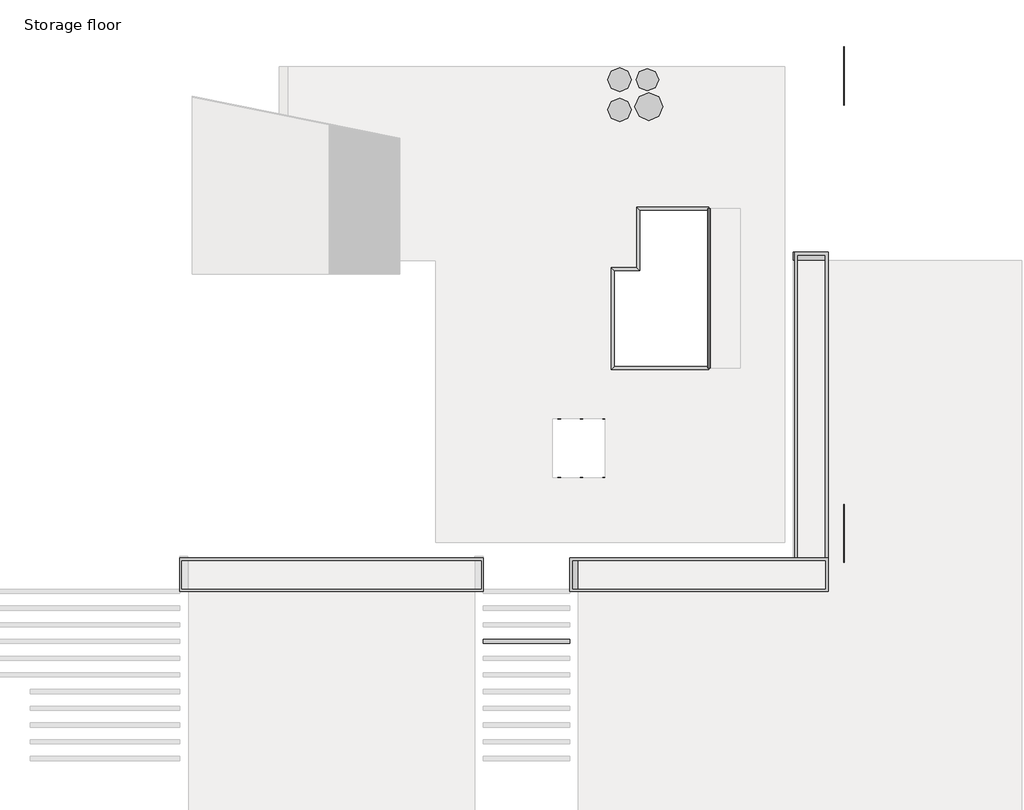
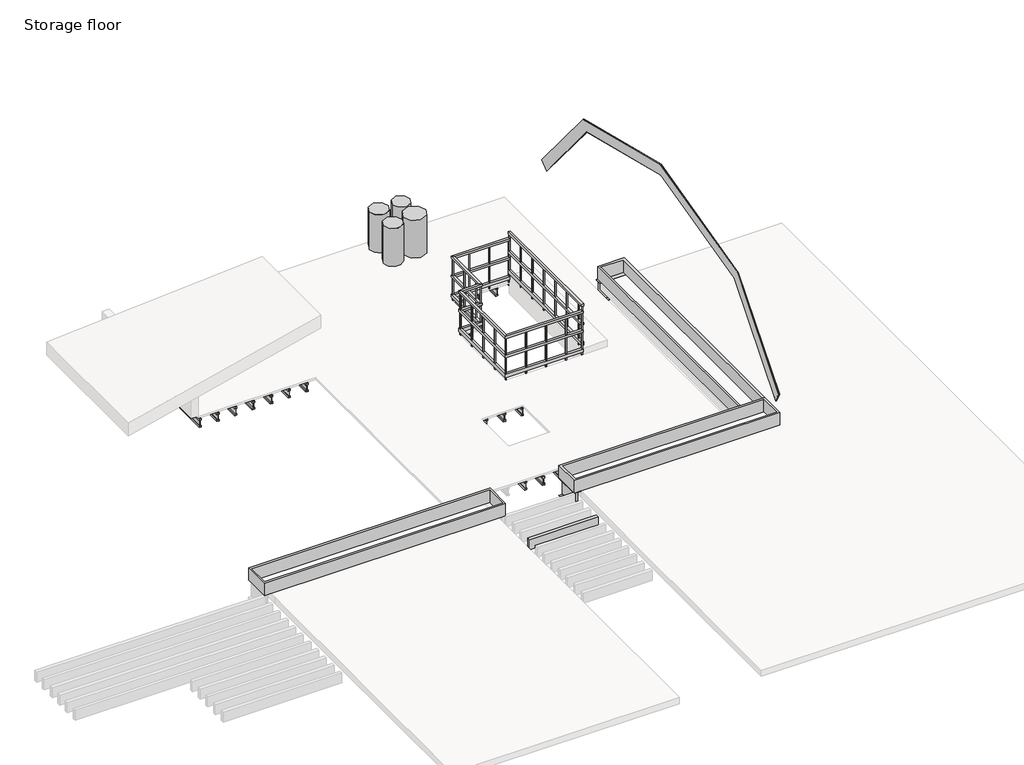
# One storey, part 2 of 2: 29 beams, 9 proxies, 2 railings.
"""IFC4 building model written with IfcOpenShell, lengths in millimetres."""

import ifcopenshell
import ifcopenshell.guid

model = None  # the IFC model being written
_history = None  # IfcOwnerHistory: only IFC2X3 demands one
_inside = {}  # id of a spatial element -> (the spatial element, [elements in it])
_under = {}  # id of a project, library or spatial element -> (it, [spatial elements below it])
_declared = {}  # id of a project -> (the project, [libraries it declares])
_typed = {}  # id of a type object -> (the type object, [elements of that type])
_made_of = {}  # id of a material, layer set ... -> (it, [elements and type objects made of it])


def new_model(schema):
    """Start an empty IFC model of exactly this schema.

    Asked for "IFC4X3", IfcOpenShell would pick the latest addendum, in which some entities
    have other attributes; the version numbers below select the first issue.
    IFC2X3 requires an IfcOwnerHistory on every rooted entity: one is made here for all.
    """
    global model, _history
    if schema == "IFC4X3":
        model = ifcopenshell.file(schema_version=(4, 3, 0, 0))
    else:
        model = ifcopenshell.file(schema=schema)
    _inside.clear()
    _under.clear()
    _declared.clear()
    _typed.clear()
    _made_of.clear()
    _history = None
    if model.schema == "IFC2X3":
        org = make("IfcOrganization", Name="unknown")
        user = make(
            "IfcPersonAndOrganization",
            ThePerson=make("IfcPerson", FamilyName="unknown"),
            TheOrganization=org,
        )
        app = make(
            "IfcApplication",
            ApplicationDeveloper=org,
            Version="unknown",
            ApplicationFullName="unknown",
            ApplicationIdentifier="unknown",
        )
        _history = make(
            "IfcOwnerHistory",
            OwningUser=user,
            OwningApplication=app,
            ChangeAction="ADDED",
            CreationDate=0,
        )
    return model


def make(cls, **values):
    """One entity of the class cls with the attributes given. An attribute that is None is left unset."""
    return model.create_entity(
        cls, **{name: value for name, value in values.items() if value is not None}
    )


def rooted(cls, **values):
    """An entity with a GlobalId (a new one), such as an element, a storey or a relation."""
    return make(cls, GlobalId=ifcopenshell.guid.new(), OwnerHistory=_history, **values)


def si_unit(unit_type, name, prefix=None):
    """IfcSIUnit, for example si_unit("LENGTHUNIT", "METRE", prefix="MILLI")."""
    return make("IfcSIUnit", UnitType=unit_type, Prefix=prefix, Name=name)


def assignment(units):
    """IfcUnitAssignment: the units of a project."""
    return None if units is None else make("IfcUnitAssignment", Units=units)


def point(xyz):
    """IfcCartesianPoint."""
    return None if xyz is None else make("IfcCartesianPoint", Coordinates=xyz)


def direction(xyz):
    """IfcDirection."""
    return None if xyz is None else make("IfcDirection", DirectionRatios=xyz)


def frame(location, z_axis=None, x_axis=None):
    """IfcAxis2Placement3D, a coordinate frame: its origin and axes. An axis left out is left unset."""
    return make(
        "IfcAxis2Placement3D",
        Location=point(location),
        Axis=direction(z_axis),
        RefDirection=direction(x_axis),
    )


def frame_2d(location, x_axis=None):
    """IfcAxis2Placement2D, a coordinate frame in the plane: its origin and x axis."""
    return make(
        "IfcAxis2Placement2D", Location=point(location), RefDirection=direction(x_axis)
    )


def origin():
    """The frame at (0, 0, 0) with its axes left unset."""
    return frame((0.0, 0.0, 0.0))


def place(relative_to, where):
    """IfcLocalPlacement: puts the frame where relative to a parent placement (None: the world)."""
    return make(
        "IfcLocalPlacement", PlacementRelTo=relative_to, RelativePlacement=where
    )


def context(
    kind, dimensions, precision=None, world=None, true_north=None, identifier=None
):
    """IfcGeometricRepresentationContext, for example the 3D "Model" context."""
    return make(
        "IfcGeometricRepresentationContext",
        ContextIdentifier=identifier,
        ContextType=kind,
        CoordinateSpaceDimension=dimensions,
        Precision=precision,
        WorldCoordinateSystem=world,
        TrueNorth=true_north,
    )


def project(units=None, contexts=None):
    """IfcProject with its units and contexts."""
    return rooted(
        "IfcProject",
        Name="project",
        RepresentationContexts=contexts,
        UnitsInContext=assignment(units),
    )


def spatial(cls, under=None, at=None, **own):
    """A site, building, storey or space (cls), placed at a placement, below another one or the project."""
    s = rooted(cls, ObjectPlacement=at, **own)
    if under is not None:
        _under.setdefault(under.id(), (under, []))[1].append(s)
    return s


def polyline(points):
    """IfcPolyline through the points."""
    return make("IfcPolyline", Points=[point(p) for p in points])


def circle_curve(where, radius):
    """IfcCircle in the frame where."""
    return make("IfcCircle", Position=where, Radius=radius)


def trimmed(basis, trim1, trim2, sense, master):
    """IfcTrimmedCurve: the piece of a basis curve between two trims."""
    return make(
        "IfcTrimmedCurve",
        BasisCurve=basis,
        Trim1=trim1,
        Trim2=trim2,
        SenseAgreement=sense,
        MasterRepresentation=master,
    )


def segment(curve, same_sense, transition):
    """IfcCompositeCurveSegment."""
    return make(
        "IfcCompositeCurveSegment",
        Transition=transition,
        SameSense=same_sense,
        ParentCurve=curve,
    )


def composite_curve(segments, self_intersect=None):
    """IfcCompositeCurve: segments joined end to end."""
    return make("IfcCompositeCurve", Segments=segments, SelfIntersect=self_intersect)


def outline(outer, holes=None, kind="AREA"):
    """IfcArbitraryClosedProfileDef: a profile drawn as a closed curve; with holes, ...WithVoids."""
    if holes is None:
        return make("IfcArbitraryClosedProfileDef", ProfileType=kind, OuterCurve=outer)
    return make(
        "IfcArbitraryProfileDefWithVoids",
        ProfileType=kind,
        OuterCurve=outer,
        InnerCurves=holes,
    )


def extrude(swept, where, along, depth):
    """IfcExtrudedAreaSolid: the profile swept, set in the frame where, extruded along a direction by depth."""
    return make(
        "IfcExtrudedAreaSolid",
        SweptArea=swept,
        Position=where,
        ExtrudedDirection=direction(along),
        Depth=depth,
    )


def faces_of(points, faces, orient=None, outer=None):
    """IfcFace entities. A face is a list of loops; a loop is a list of indices into points, from 0.

    orient and outer hold one flag for each loop. By default every Orientation is true, the
    first loop of a face is its IfcFaceOuterBound and the others are IfcFaceBound.
    """
    made = []
    for i, loops in enumerate(faces):
        bounds = []
        for j, loop in enumerate(loops):
            is_outer = j == 0 if outer is None else outer[i][j]
            bounds.append(
                make(
                    "IfcFaceOuterBound" if is_outer else "IfcFaceBound",
                    Bound=make("IfcPolyLoop", Polygon=[points[k] for k in loop]),
                    Orientation=True if orient is None else orient[i][j],
                )
            )
        made.append(make("IfcFace", Bounds=bounds))
    return made


def faceted_brep(points, faces, orient=None, outer=None, voids=None):
    """IfcFacetedBrep: a solid bounded by flat faces; with voids (closed shells), ...WithVoids."""
    shared = [point(p) for p in points]
    hull = make("IfcClosedShell", CfsFaces=faces_of(shared, faces, orient, outer))
    if voids is None:
        return make("IfcFacetedBrep", Outer=hull)
    return make(
        "IfcFacetedBrepWithVoids",
        Outer=hull,
        Voids=[
            make(cls, CfsFaces=faces_of(shared, fs, o, b)) for cls, fs, o, b in voids
        ],
    )


def shape(context_of_items, identifier, shape_type, items):
    """IfcShapeRepresentation: the items that make up one representation, for example the "Body"."""
    return make(
        "IfcShapeRepresentation",
        ContextOfItems=context_of_items,
        RepresentationIdentifier=identifier,
        RepresentationType=shape_type,
        Items=items,
    )


def source(mapping_origin, context_of_items, identifier, shape_type, items):
    """IfcRepresentationMap: a shape defined once, which mapped items show again and again."""
    return make(
        "IfcRepresentationMap",
        MappingOrigin=mapping_origin,
        MappedRepresentation=shape(context_of_items, identifier, shape_type, items),
    )


def transform(
    local_origin,
    x_axis=None,
    y_axis=None,
    z_axis=None,
    scale=None,
    scale2=None,
    scale3=None,
    uniform=True,
):
    """IfcCartesianTransformationOperator3D, or its non-uniform kind. x_axis, y_axis, z_axis: its Axis1, 2, 3."""
    if uniform:
        return make(
            "IfcCartesianTransformationOperator3D",
            Axis1=direction(x_axis),
            Axis2=direction(y_axis),
            LocalOrigin=point(local_origin),
            Scale=scale,
            Axis3=direction(z_axis),
        )
    return make(
        "IfcCartesianTransformationOperator3DnonUniform",
        Axis1=direction(x_axis),
        Axis2=direction(y_axis),
        LocalOrigin=point(local_origin),
        Scale=scale,
        Axis3=direction(z_axis),
        Scale2=scale2,
        Scale3=scale3,
    )


def mapped(mapping_source, mapping_target):
    """IfcMappedItem: shows the shape of a source again, moved by a transform."""
    return make(
        "IfcMappedItem", MappingSource=mapping_source, MappingTarget=mapping_target
    )


def made_of(thing, what):
    """Note that an element or type object is made of a material, layer set ...; save() writes the relation."""
    if what is not None:
        _made_of.setdefault(what.id(), (what, []))[1].append(thing)
    return thing


def element(
    cls,
    number,
    at=None,
    inside=None,
    cuts=None,
    type_object=None,
    material=None,
    context=None,
    identifier="Body",
    shape_type=None,
    held_by="IfcProductDefinitionShape",
    body=None,
    shapes=None,
    **own,
):
    """One element of the class cls, such as IfcWall. Its Tag is "e" and its number.

    at: its placement. inside: the storey or other place that contains it. cuts: it is an
    opening in that element (IfcRelVoidsElement). A single representation is given by context,
    identifier, shape_type and body (its items); several are given by shapes. held_by: the class
    of the entity that holds the representations. save() writes the other relations.
    """
    e = rooted(cls, Tag="e%d" % number, ObjectPlacement=at, **own)
    if body is not None:
        shapes = [shape(context, identifier, shape_type, body)]
    if shapes is not None:
        e.Representation = make(held_by, Representations=shapes)
    if inside is not None:
        _inside.setdefault(inside.id(), (inside, []))[1].append(e)
    if cuts is not None:
        rooted(
            "IfcRelVoidsElement", RelatingBuildingElement=cuts, RelatedOpeningElement=e
        )
    if type_object is not None:
        _typed.setdefault(type_object.id(), (type_object, []))[1].append(e)
    return made_of(e, material)


def aggregate(whole, parts):
    """IfcRelAggregates: a whole, such as a stair, and the parts it consists of."""
    return rooted("IfcRelAggregates", RelatingObject=whole, RelatedObjects=parts)


def save(model, path):
    """Write the relations noted so far, then the file.

    IfcRelAggregates (storeys below a building ...), IfcRelContainedInSpatialStructure (elements
    in a storey), IfcRelDefinesByType, IfcRelAssociatesMaterial and IfcRelDeclares: one each for
    every whole, place, type object, material and project.
    """
    for whole, parts in _under.values():
        aggregate(whole, parts)
    for where, things in _inside.values():
        rooted(
            "IfcRelContainedInSpatialStructure",
            RelatedElements=things,
            RelatingStructure=where,
        )
    for kind, things in _typed.values():
        rooted("IfcRelDefinesByType", RelatedObjects=things, RelatingType=kind)
    for what, things in _made_of.values():
        rooted("IfcRelAssociatesMaterial", RelatedObjects=things, RelatingMaterial=what)
    for by, libraries in _declared.values():
        rooted("IfcRelDeclares", RelatingContext=by, RelatedDefinitions=libraries)
    model.write(path)


def plywood_web_joist_2_x_8_7c958bd9(model_context):
    return source(origin(), model_context, "Body", "SweptSolid", [
        extrude(outline(polyline([(-25.4, 101.6), (25.4, 101.6), (25.4, 63.5), (4.7625, 63.5), (4.7625, 69.85), (-4.7625, 69.85), (-4.7625, 63.5), (-25.4, 63.5), (-25.4, 101.6)])), frame((-4318.0, 0.0, 0.0), z_axis=(1.0, 0.0, 0.0), x_axis=(0.0, 1.0, 0.0)), (0.0, 0.0, 1.0), 8636.0),
        extrude(outline(polyline([(25.4, -63.5), (25.4, -101.6), (-25.4, -101.6), (-25.4, -63.5), (-4.7625, -63.5), (-4.7625, -69.1160374), (4.7625, -69.1160374), (4.7625, -63.5), (25.4, -63.5)])), frame((-4318.0, 0.0, 0.0), z_axis=(1.0, 0.0, 0.0), x_axis=(0.0, 1.0, 0.0)), (0.0, 0.0, 1.0), 8636.0),
        extrude(outline(polyline([(4318.0, 4.7625), (4318.0, -4.7625), (-4318.0, -4.7625), (-4318.0, 4.7625), (4318.0, 4.7625)])), frame((0.0, 0.0, -69.1160374), z_axis=(0.0, 0.0, 1.0), x_axis=(1.0, 0.0, 0.0)), (0.0, 0.0, 1.0), 138.9660374),
    ])


def plywood_web_joist_2_x_8_e6685f11(model_context):
    return source(origin(), model_context, "Body", "SweptSolid", [
        extrude(outline(polyline([(-25.4, 101.6), (25.4, 101.6), (25.4, 63.5), (4.7625, 63.5), (4.7625, 69.85), (-4.7625, 69.85), (-4.7625, 63.5), (-25.4, 63.5), (-25.4, 101.6)])), frame((-1284.2875, 0.0, 0.0), z_axis=(1.0, 0.0, 0.0), x_axis=(0.0, 1.0, 0.0)), (0.0, 0.0, 1.0), 2568.575),
        extrude(outline(polyline([(25.4, -63.5), (25.4, -101.6), (-25.4, -101.6), (-25.4, -63.5), (-4.7625, -63.5), (-4.7625, -69.1160374), (4.7625, -69.1160374), (4.7625, -63.5), (25.4, -63.5)])), frame((-1284.2875, 0.0, 0.0), z_axis=(1.0, 0.0, 0.0), x_axis=(0.0, 1.0, 0.0)), (0.0, 0.0, 1.0), 2568.575),
        extrude(outline(polyline([(1284.2875, 4.7625), (1284.2875, -4.7625), (-1284.2875, -4.7625), (-1284.2875, 4.7625), (1284.2875, 4.7625)])), frame((0.0, 0.0, -69.1160374), z_axis=(0.0, 0.0, 1.0), x_axis=(1.0, 0.0, 0.0)), (0.0, 0.0, 1.0), 138.9660374),
    ])


def plywood_web_joist_2_x_8_5f52603e(model_context):
    return source(origin(), model_context, "Body", "SweptSolid", [
        extrude(outline(polyline([(-25.4, 101.6), (25.4, 101.6), (25.4, 63.5), (4.7625, 63.5), (4.7625, 69.85), (-4.7625, 69.85), (-4.7625, 63.5), (-25.4, 63.5), (-25.4, 101.6)])), frame((-1584.325, 0.0, 0.0), z_axis=(1.0, 0.0, 0.0), x_axis=(0.0, 1.0, 0.0)), (0.0, 0.0, 1.0), 3168.65),
        extrude(outline(polyline([(25.4, -63.5), (25.4, -101.6), (-25.4, -101.6), (-25.4, -63.5), (-4.7625, -63.5), (-4.7625, -69.1160374), (4.7625, -69.1160374), (4.7625, -63.5), (25.4, -63.5)])), frame((-1584.325, 0.0, 0.0), z_axis=(1.0, 0.0, 0.0), x_axis=(0.0, 1.0, 0.0)), (0.0, 0.0, 1.0), 3168.65),
        extrude(outline(polyline([(1584.325, 4.7625), (1584.325, -4.7625), (-1584.325, -4.7625), (-1584.325, 4.7625), (1584.325, 4.7625)])), frame((0.0, 0.0, -69.1160374), z_axis=(0.0, 0.0, 1.0), x_axis=(1.0, 0.0, 0.0)), (0.0, 0.0, 1.0), 138.9660374),
    ])


def plywood_web_joist_2_x_8_093a3c26(model_context):
    return source(origin(), model_context, "Body", "SweptSolid", [
        extrude(outline(polyline([(-25.4, 101.6), (25.4, 101.6), (25.4, 63.5), (4.7625, 63.5), (4.7625, 69.85), (-4.7625, 69.85), (-4.7625, 63.5), (-25.4, 63.5), (-25.4, 101.6)])), frame((-1835.15, 0.0, 0.0), z_axis=(1.0, 0.0, 0.0), x_axis=(0.0, 1.0, 0.0)), (0.0, 0.0, 1.0), 3670.3),
        extrude(outline(polyline([(25.4, -63.5), (25.4, -101.6), (-25.4, -101.6), (-25.4, -63.5), (-4.7625, -63.5), (-4.7625, -69.1160374), (4.7625, -69.1160374), (4.7625, -63.5), (25.4, -63.5)])), frame((-1835.15, 0.0, 0.0), z_axis=(1.0, 0.0, 0.0), x_axis=(0.0, 1.0, 0.0)), (0.0, 0.0, 1.0), 3670.3),
        extrude(outline(polyline([(1835.15, 4.7625), (1835.15, -4.7625), (-1835.15, -4.7625), (-1835.15, 4.7625), (1835.15, 4.7625)])), frame((0.0, 0.0, -69.1160374), z_axis=(0.0, 0.0, 1.0), x_axis=(1.0, 0.0, 0.0)), (0.0, 0.0, 1.0), 138.9660374),
    ])


def plywood_web_joist_2_x_8_156d774c(model_context):
    return source(origin(), model_context, "Body", "SweptSolid", [
        extrude(outline(polyline([(-25.4, 101.6), (25.4, 101.6), (25.4, 63.5), (4.7625, 63.5), (4.7625, 69.85), (-4.7625, 69.85), (-4.7625, 63.5), (-25.4, 63.5), (-25.4, 101.6)])), frame((-3195.5616975, 0.0, 0.0), z_axis=(1.0, 0.0, 0.0), x_axis=(0.0, 1.0, 0.0)), (0.0, 0.0, 1.0), 6391.1233951),
        extrude(outline(polyline([(25.4, -63.5), (25.4, -101.6), (-25.4, -101.6), (-25.4, -63.5), (-4.7625, -63.5), (-4.7625, -69.1160374), (4.7625, -69.1160374), (4.7625, -63.5), (25.4, -63.5)])), frame((-3195.5616975, 0.0, 0.0), z_axis=(1.0, 0.0, 0.0), x_axis=(0.0, 1.0, 0.0)), (0.0, 0.0, 1.0), 6391.1233951),
        extrude(outline(polyline([(3195.5616975, 4.7625), (3195.5616975, -4.7625), (-3195.5616975, -4.7625), (-3195.5616975, 4.7625), (3195.5616975, 4.7625)])), frame((0.0, 0.0, -69.1160374), z_axis=(0.0, 0.0, 1.0), x_axis=(1.0, 0.0, 0.0)), (0.0, 0.0, 1.0), 138.9660374),
    ])


def plywood_web_joist_2_x_8_69fe57bf(model_context):
    return source(origin(), model_context, "Body", "SweptSolid", [
        extrude(outline(polyline([(-25.4, 101.6), (25.4, 101.6), (25.4, 63.5), (4.7625, 63.5), (4.7625, 69.85), (-4.7625, 69.85), (-4.7625, 63.5), (-25.4, 63.5), (-25.4, 101.6)])), frame((-589.0383025, 0.0, 0.0), z_axis=(1.0, 0.0, 0.0), x_axis=(0.0, 1.0, 0.0)), (0.0, 0.0, 1.0), 1178.0766049),
        extrude(outline(polyline([(25.4, -63.5), (25.4, -101.6), (-25.4, -101.6), (-25.4, -63.5), (-4.7625, -63.5), (-4.7625, -69.1160374), (4.7625, -69.1160374), (4.7625, -63.5), (25.4, -63.5)])), frame((-589.0383025, 0.0, 0.0), z_axis=(1.0, 0.0, 0.0), x_axis=(0.0, 1.0, 0.0)), (0.0, 0.0, 1.0), 1178.0766049),
        extrude(outline(polyline([(589.0383025, 4.7625), (589.0383025, -4.7625), (-589.0383025, -4.7625), (-589.0383025, 4.7625), (589.0383025, 4.7625)])), frame((0.0, 0.0, -69.1160374), z_axis=(0.0, 0.0, 1.0), x_axis=(1.0, 0.0, 0.0)), (0.0, 0.0, 1.0), 138.9660374),
    ])


def plywood_web_joist_2_x_8_8e4157b3(model_context):
    return source(origin(), model_context, "Body", "SweptSolid", [
        extrude(outline(polyline([(-25.4, 101.6), (25.4, 101.6), (25.4, 63.5), (4.7625, 63.5), (4.7625, 69.85), (-4.7625, 69.85), (-4.7625, 63.5), (-25.4, 63.5), (-25.4, 101.6)])), frame((-1758.95, 0.0, 0.0), z_axis=(1.0, 0.0, 0.0), x_axis=(0.0, 1.0, 0.0)), (0.0, 0.0, 1.0), 3517.9),
        extrude(outline(polyline([(25.4, -63.5), (25.4, -101.6), (-25.4, -101.6), (-25.4, -63.5), (-4.7625, -63.5), (-4.7625, -69.1160374), (4.7625, -69.1160374), (4.7625, -63.5), (25.4, -63.5)])), frame((-1758.95, 0.0, 0.0), z_axis=(1.0, 0.0, 0.0), x_axis=(0.0, 1.0, 0.0)), (0.0, 0.0, 1.0), 3517.9),
        extrude(outline(polyline([(1758.95, 4.7625), (1758.95, -4.7625), (-1758.95, -4.7625), (-1758.95, 4.7625), (1758.95, 4.7625)])), frame((0.0, 0.0, -69.1160374), z_axis=(0.0, 0.0, 1.0), x_axis=(1.0, 0.0, 0.0)), (0.0, 0.0, 1.0), 138.9660374),
    ])


def timber_3x10_88a0bdfd(model_context):
    return source(origin(), model_context, "Body", "SweptSolid", [
        extrude(outline(polyline([(785.1325751, 38.1), (785.1325751, -38.1), (-785.1325751, -38.1), (-785.1325751, 38.1), (785.1325751, 38.1)])), frame((0.0, 0.0, -120.65), z_axis=(0.0, 0.0, 1.0), x_axis=(1.0, 0.0, 0.0)), (0.0, 0.0, 1.0), 241.3),
    ])


def w_shapes_w_6x16_3_4_ba0ed1b2(model_context):
    return source(origin(), model_context, "Body", "SweptSolid", [
        extrude(outline(composite_curve([segment(polyline([(76.1964281, -203.073), (76.1964281, -212.725), (-76.2035719, -212.725), (-76.2035719, -203.073), (-10.5445719, -203.073)]), True, "CONTINUOUS"), segment(trimmed(circle_curve(frame_2d((-10.5445719, -195.453)), 7.62), [point((-10.5445719, -203.073))], [point((-2.9245719, -195.453))], True, "CARTESIAN"), True, "CONTINUOUS"), segment(polyline([(-2.9245719, -195.453), (-2.9245719, 195.453)]), True, "CONTINUOUS"), segment(trimmed(circle_curve(frame_2d((-10.5445719, 195.453)), 7.62), [point((-2.9245719, 195.453))], [point((-10.5445719, 203.073))], True, "CARTESIAN"), True, "CONTINUOUS"), segment(polyline([(-10.5445719, 203.073), (-76.2035719, 203.073), (-76.2035719, 212.725), (76.1964281, 212.725), (76.1964281, 203.073), (10.5374281, 203.073)]), True, "CONTINUOUS"), segment(trimmed(circle_curve(frame_2d((10.5374281, 195.453)), 7.62), [point((10.5374281, 203.073))], [point((2.9174281, 195.453))], True, "CARTESIAN"), True, "CONTINUOUS"), segment(polyline([(2.9174281, 195.453), (2.9174281, -195.453)]), True, "CONTINUOUS"), segment(trimmed(circle_curve(frame_2d((10.5374281, -195.453)), 7.62), [point((2.9174281, -195.453))], [point((10.5374281, -203.073))], True, "CARTESIAN"), True, "CONTINUOUS"), segment(polyline([(10.5374281, -203.073), (76.1964281, -203.073)]), True, "CONTINUOUS")], self_intersect=False)), frame((-303.1556375, 0.0, 0.0), z_axis=(1.0, 0.0, 0.0), x_axis=(0.0, 1.0, 0.0)), (0.0, 0.0, 1.0), 606.311275),
    ])


def w_shapes_w_6x18_5_26640f6b(model_context):
    return source(origin(), model_context, "Body", "SweptSolid", [
        extrude(outline(composite_curve([segment(polyline([(76.1964281, -225.298), (76.1964281, -234.95), (-76.2035719, -234.95), (-76.2035719, -225.298), (-10.5445719, -225.298)]), True, "CONTINUOUS"), segment(trimmed(circle_curve(frame_2d((-10.5445719, -217.678)), 7.62), [point((-10.5445719, -225.298))], [point((-2.9245719, -217.678))], True, "CARTESIAN"), True, "CONTINUOUS"), segment(polyline([(-2.9245719, -217.678), (-2.9245719, 217.678)]), True, "CONTINUOUS"), segment(trimmed(circle_curve(frame_2d((-10.5445719, 217.678)), 7.62), [point((-2.9245719, 217.678))], [point((-10.5445719, 225.298))], True, "CARTESIAN"), True, "CONTINUOUS"), segment(polyline([(-10.5445719, 225.298), (-76.2035719, 225.298), (-76.2035719, 234.95), (76.1964281, 234.95), (76.1964281, 225.298), (10.5374281, 225.298)]), True, "CONTINUOUS"), segment(trimmed(circle_curve(frame_2d((10.5374281, 217.678)), 7.62), [point((10.5374281, 225.298))], [point((2.9174281, 217.678))], True, "CARTESIAN"), True, "CONTINUOUS"), segment(polyline([(2.9174281, 217.678), (2.9174281, -217.678)]), True, "CONTINUOUS"), segment(trimmed(circle_curve(frame_2d((10.5374281, -217.678)), 7.62), [point((2.9174281, -217.678))], [point((10.5374281, -225.298))], True, "CARTESIAN"), True, "CONTINUOUS"), segment(polyline([(10.5374281, -225.298), (76.1964281, -225.298)]), True, "CONTINUOUS")], self_intersect=False)), frame((-317.5, 0.0, 0.0), z_axis=(1.0, 0.0, 0.0), x_axis=(0.0, 1.0, 0.0)), (0.0, 0.0, 1.0), 635.0),
    ])


def generic_models_2_generic_models_1_059ed1a1(model_context):
    return source(origin(), model_context, "Body", "SweptSolid", [
        extrude(outline(polyline([(11609.9309883, 2984.3405795), (10023.6412719, 4887.8882391), (7113.0570149, 5615.5343034), (4202.4384941, 4887.8796732), (2560.7151338, 2917.8116409), (2434.8673967, 3148.0206952), (4066.3626163, 5105.8149588), (7113.772024, 5867.6673107), (10161.1814316, 5105.8149588), (11797.360301, 3142.4003155), (11609.9309883, 2984.3405795)])), frame((29947.3870052, 0.0, 0.0), z_axis=(1.0, 0.0, 0.0), x_axis=(0.0, 1.0, 0.0)), (0.0, 0.0, 1.0), 13.5023771),
    ])


def generic_models_4_generic_models_1_4f2df183(model_context):
    return source(origin(), model_context, "Body", "SweptSolid", [
        extrude(outline(polyline([(11606.2878096, 2984.3405795), (10019.9980933, 4887.8882391), (7109.4138362, 5615.5343034), (4198.7953154, 4887.8796732), (2604.5089175, 2974.7359957), (2431.2242181, 3148.0206952), (4062.7194377, 5105.8149588), (7110.1288453, 5867.6673107), (10157.5382529, 5105.8149588), (11793.7171223, 3142.4003155), (11606.2878096, 2984.3405795)])), frame((29947.3870052, 0.0, 0.0), z_axis=(1.0, 0.0, 0.0), x_axis=(0.0, 1.0, 0.0)), (0.0, 0.0, 1.0), 13.5023771),
    ])


def press_tank_press_tank_b5f43448(model_context):
    return source(origin(), model_context, "Body", "SweptSolid", [
        extrude(outline(composite_curve([segment(trimmed(circle_curve(frame_2d((23819.6370052, 10524.1286841)), 203.2), [point((23616.4370052, 10524.1286841))], [point((24022.8370052, 10524.1286841))], False, "CARTESIAN"), True, "CONTINUOUS"), segment(trimmed(circle_curve(frame_2d((23819.6370052, 10524.1286841)), 203.2), [point((24022.8370052, 10524.1286841))], [point((23616.4370052, 10524.1286841))], False, "CARTESIAN"), True, "CONTINUOUS")], self_intersect=False)), frame((0.0, 0.0, 2832.1), z_axis=(0.0, 0.0, 1.0), x_axis=(1.0, 0.0, 0.0)), (0.0, 0.0, 1.0), 914.4),
    ])


def press_tank1_press_tank_732dd890(model_context):
    return source(origin(), model_context, "Body", "SweptSolid", [
        extrude(outline(composite_curve([segment(trimmed(circle_curve(frame_2d((26385.9004782, 10738.3240491)), 254.0), [point((26131.9004782, 10738.3240491))], [point((26639.9004782, 10738.3240491))], False, "CARTESIAN"), True, "CONTINUOUS"), segment(trimmed(circle_curve(frame_2d((26385.9004782, 10738.3240491)), 254.0), [point((26639.9004782, 10738.3240491))], [point((26131.9004782, 10738.3240491))], False, "CARTESIAN"), True, "CONTINUOUS")], self_intersect=False)), frame((0.0, 0.0, 2832.1), z_axis=(0.0, 0.0, 1.0), x_axis=(1.0, 0.0, 0.0)), (0.0, 0.0, 1.0), 914.4),
    ])


def water_boiler_water_boiler_54bea4d4(model_context):
    return source(origin(), model_context, "Body", "SweptSolid", [
        extrude(outline(composite_curve([segment(trimmed(circle_curve(frame_2d((25724.6370052, 10998.0325125)), 215.9), [point((25508.7370052, 10998.0325125))], [point((25940.5370052, 10998.0325125))], False, "CARTESIAN"), True, "CONTINUOUS"), segment(trimmed(circle_curve(frame_2d((25724.6370052, 10998.0325125)), 215.9), [point((25940.5370052, 10998.0325125))], [point((25508.7370052, 10998.0325125))], False, "CARTESIAN"), True, "CONTINUOUS")], self_intersect=False)), frame((0.0, 0.0, 2832.1), z_axis=(0.0, 0.0, 1.0), x_axis=(1.0, 0.0, 0.0)), (0.0, 0.0, 1.0), 914.4),
    ])


def gutter_gutter_dc17c88e(model_context):
    return source(origin(), model_context, "Body", "SweptSolid", [
        extrude(outline(polyline([(23406.8870052, 1909.5502616), (17901.4334333, 1909.5502616), (17901.4334333, 2515.8615366), (23406.8870052, 2515.8615366), (23406.8870052, 1909.5502616)]), holes=[polyline([(23370.1856701, 2465.0615366), (17939.5370052, 2465.0615366), (17939.5370052, 1956.0872459), (23370.1856701, 1956.0872459), (23370.1856701, 2465.0615366)])]), frame((0.0, 0.0, 2832.1), z_axis=(0.0, 0.0, 1.0), x_axis=(1.0, 0.0, 0.0)), (0.0, 0.0, 1.0), 304.8),
    ])


def gutter1_gutter_22c69523(model_context):
    return source(origin(), model_context, "Body", "SweptSolid", [
        extrude(outline(polyline([(29665.9107095, 1909.5502616), (24977.1521553, 1909.5502616), (24977.1521553, 2515.8615366), (29665.9107095, 2515.8615366), (29665.9107095, 1909.5502616)]), holes=[polyline([(29616.401408, 2465.0615366), (25031.5521553, 2465.0615366), (25031.5521553, 1956.0872459), (29616.401408, 1956.0872459), (29616.401408, 2465.0615366)])]), frame((0.0, 0.0, 2832.1), z_axis=(0.0, 0.0, 1.0), x_axis=(1.0, 0.0, 0.0)), (0.0, 0.0, 1.0), 304.8),
    ])


def gutter2_gutter_d7d01a53(model_context):
    return source(origin(), model_context, "Body", "SweptSolid", [
        extrude(outline(polyline([(29060.890133, 2515.8615366), (29060.890133, 8064.3148819), (29667.201408, 8064.3148819), (29667.201408, 2515.8615366), (29616.401408, 2515.8615366), (29616.401408, 8009.9148819), (29107.4271173, 8009.9148819), (29107.4271173, 2515.8615366), (29060.890133, 2515.8615366)])), frame((0.0, 0.0, 2832.1), z_axis=(0.0, 0.0, 1.0), x_axis=(1.0, 0.0, 0.0)), (0.0, 0.0, 1.0), 304.8),
    ])


model = new_model("IFC4")

# Units and contexts
model_context = context("Model", 3, world=origin())
ifc_project = project(units=[si_unit("LENGTHUNIT", "METRE", prefix="MILLI")], contexts=[model_context])

# Site, building, storey
site = spatial("IfcSite", under=ifc_project)
building = spatial("IfcBuilding", under=site)
storey = spatial("IfcBuildingStorey", under=building, Name="Storage floor", Elevation=2832.1)

# Beams
placement = place(None, origin())
plywood_web_joist_2_x_8_shape = plywood_web_joist_2_x_8_7c958bd9(model_context)
element("IfcBeam", 1, ObjectType="Plywood Web Joist : 2 x 8", at=placement, inside=storey, context=model_context, shape_type="MappedRepresentation", body=[
    mapped(plywood_web_joist_2_x_8_shape, transform((28850.8792207, 7113.2615366, 2686.05), x_axis=(0.0, -1.0, 0.0), y_axis=(1.0, 0.0, 0.0), z_axis=(0.0, 0.0, 1.0))),
])
element("IfcBeam", 2, ObjectType="Plywood Web Joist : 2 x 8", at=placement, inside=storey, context=model_context, shape_type="MappedRepresentation", body=[
    mapped(plywood_web_joist_2_x_8_shape, transform((28444.4792207, 7113.2615366, 2686.05), x_axis=(0.0, -1.0, 0.0), y_axis=(1.0, 0.0, 0.0), z_axis=(0.0, 0.0, 1.0))),
])
element("IfcBeam", 3, ObjectType="Plywood Web Joist : 2 x 8", at=placement, inside=storey, context=model_context, shape_type="MappedRepresentation", body=[
    mapped(plywood_web_joist_2_x_8_shape, transform((28038.0792207, 7113.2615366, 2686.05), x_axis=(0.0, -1.0, 0.0), y_axis=(1.0, 0.0, 0.0), z_axis=(0.0, 0.0, 1.0))),
])
element("IfcBeam", 4, ObjectType="Plywood Web Joist : 2 x 8", at=placement, inside=storey, context=model_context, shape_type="MappedRepresentation", body=[
    mapped(plywood_web_joist_2_x_8_shape, transform((27631.6792207, 7113.2615366, 2686.05), x_axis=(0.0, -1.0, 0.0), y_axis=(1.0, 0.0, 0.0), z_axis=(0.0, 0.0, 1.0))),
])
element("IfcBeam", 5, ObjectType="Plywood Web Joist : 2 x 8", at=placement, inside=storey, context=model_context, shape_type="MappedRepresentation", body=[
    mapped(plywood_web_joist_2_x_8_shape, transform((24380.4792207, 7113.2615366, 2686.05), x_axis=(0.0, -1.0, 0.0), y_axis=(1.0, 0.0, 0.0), z_axis=(0.0, 0.0, 1.0))),
])
plywood_web_joist_2_x_8_2_shape = plywood_web_joist_2_x_8_e6685f11(model_context)
element("IfcBeam", 6, ObjectType="Plywood Web Joist : 2 x 8", at=placement, inside=storey, context=model_context, shape_type="MappedRepresentation", body=[
    mapped(plywood_web_joist_2_x_8_2_shape, transform((27225.2792207, 10146.9740366, 2686.05), x_axis=(0.0, -1.0, 0.0), y_axis=(1.0, 0.0, 0.0), z_axis=(0.0, 0.0, 1.0))),
])
element("IfcBeam", 7, ObjectType="Plywood Web Joist : 2 x 8", at=placement, inside=storey, context=model_context, shape_type="MappedRepresentation", body=[
    mapped(plywood_web_joist_2_x_8_2_shape, transform((26818.8792207, 10146.9740366, 2686.05), x_axis=(0.0, -1.0, 0.0), y_axis=(1.0, 0.0, 0.0), z_axis=(0.0, 0.0, 1.0))),
])
element("IfcBeam", 8, ObjectType="Plywood Web Joist : 2 x 8", at=placement, inside=storey, context=model_context, shape_type="MappedRepresentation", body=[
    mapped(plywood_web_joist_2_x_8_2_shape, transform((26412.4792207, 10146.9740366, 2686.05), x_axis=(0.0, -1.0, 0.0), y_axis=(1.0, 0.0, 0.0), z_axis=(0.0, 0.0, 1.0))),
])
plywood_web_joist_2_x_8_3_shape = plywood_web_joist_2_x_8_5f52603e(model_context)
element("IfcBeam", 9, ObjectType="Plywood Web Joist : 2 x 8", at=placement, inside=storey, context=model_context, shape_type="MappedRepresentation", body=[
    mapped(plywood_web_joist_2_x_8_3_shape, transform((27225.2792207, 4379.5865366, 2686.05), x_axis=(0.0, -1.0, 0.0), y_axis=(1.0, 0.0, 0.0), z_axis=(0.0, 0.0, 1.0))),
])
element("IfcBeam", 10, ObjectType="Plywood Web Joist : 2 x 8", at=placement, inside=storey, context=model_context, shape_type="MappedRepresentation", body=[
    mapped(plywood_web_joist_2_x_8_3_shape, transform((26818.8792207, 4379.5865366, 2686.05), x_axis=(0.0, -1.0, 0.0), y_axis=(1.0, 0.0, 0.0), z_axis=(0.0, 0.0, 1.0))),
])
element("IfcBeam", 11, ObjectType="Plywood Web Joist : 2 x 8", at=placement, inside=storey, context=model_context, shape_type="MappedRepresentation", body=[
    mapped(plywood_web_joist_2_x_8_3_shape, transform((26412.4792207, 4379.5865366, 2686.05), x_axis=(0.0, -1.0, 0.0), y_axis=(1.0, 0.0, 0.0), z_axis=(0.0, 0.0, 1.0))),
])
element("IfcBeam", 12, ObjectType="Plywood Web Joist : 2 x 8", at=placement, inside=storey, context=model_context, shape_type="MappedRepresentation", body=[
    mapped(plywood_web_joist_2_x_8_3_shape, transform((26006.0792207, 4379.5865366, 2686.05), x_axis=(0.0, -1.0, 0.0), y_axis=(1.0, 0.0, 0.0), z_axis=(0.0, 0.0, 1.0))),
])
plywood_web_joist_2_x_8_4_shape = plywood_web_joist_2_x_8_093a3c26(model_context)
element("IfcBeam", 13, ObjectType="Plywood Web Joist : 2 x 8", at=placement, inside=storey, context=model_context, shape_type="MappedRepresentation", body=[
    mapped(plywood_web_joist_2_x_8_4_shape, transform((26006.0792207, 9596.1115366, 2686.05), x_axis=(0.0, -1.0, 0.0), y_axis=(1.0, 0.0, 0.0), z_axis=(0.0, 0.0, 1.0))),
])
plywood_web_joist_2_x_8_5_shape = plywood_web_joist_2_x_8_156d774c(model_context)
element("IfcBeam", 14, ObjectType="Plywood Web Joist : 2 x 8", at=placement, inside=storey, context=model_context, shape_type="MappedRepresentation", body=[
    mapped(plywood_web_joist_2_x_8_5_shape, transform((25599.6792207, 8235.6998391, 2686.05), x_axis=(0.0, -1.0, 0.0), y_axis=(1.0, 0.0, 0.0), z_axis=(0.0, 0.0, 1.0))),
])
element("IfcBeam", 15, ObjectType="Plywood Web Joist : 2 x 8", at=placement, inside=storey, context=model_context, shape_type="MappedRepresentation", body=[
    mapped(plywood_web_joist_2_x_8_5_shape, transform((25193.2792207, 8235.6998391, 2686.05), x_axis=(0.0, -1.0, 0.0), y_axis=(1.0, 0.0, 0.0), z_axis=(0.0, 0.0, 1.0))),
])
element("IfcBeam", 16, ObjectType="Plywood Web Joist : 2 x 8", at=placement, inside=storey, context=model_context, shape_type="MappedRepresentation", body=[
    mapped(plywood_web_joist_2_x_8_5_shape, transform((24786.8792207, 8235.6998391, 2686.05), x_axis=(0.0, -1.0, 0.0), y_axis=(1.0, 0.0, 0.0), z_axis=(0.0, 0.0, 1.0))),
])
plywood_web_joist_2_x_8_6_shape = plywood_web_joist_2_x_8_69fe57bf(model_context)
element("IfcBeam", 17, ObjectType="Plywood Web Joist : 2 x 8", at=placement, inside=storey, context=model_context, shape_type="MappedRepresentation", body=[
    mapped(plywood_web_joist_2_x_8_6_shape, transform((25599.6792207, 3384.2998391, 2657.767466), x_axis=(0.0, -1.0, 0.0), y_axis=(1.0, 0.0, 0.0), z_axis=(0.0, 0.0, 1.0))),
])
element("IfcBeam", 18, ObjectType="Plywood Web Joist : 2 x 8", at=placement, inside=storey, context=model_context, shape_type="MappedRepresentation", body=[
    mapped(plywood_web_joist_2_x_8_6_shape, transform((25193.2792207, 3384.2998391, 2657.767466), x_axis=(0.0, -1.0, 0.0), y_axis=(1.0, 0.0, 0.0), z_axis=(0.0, 0.0, 1.0))),
])
element("IfcBeam", 19, ObjectType="Plywood Web Joist : 2 x 8", at=placement, inside=storey, context=model_context, shape_type="MappedRepresentation", body=[
    mapped(plywood_web_joist_2_x_8_6_shape, transform((24786.8792207, 3384.2998391, 2657.767466), x_axis=(0.0, -1.0, 0.0), y_axis=(1.0, 0.0, 0.0), z_axis=(0.0, 0.0, 1.0))),
])
plywood_web_joist_2_x_8_7_shape = plywood_web_joist_2_x_8_8e4157b3(model_context)
element("IfcBeam", 20, ObjectType="Plywood Web Joist : 2 x 8", at=placement, inside=storey, context=model_context, shape_type="MappedRepresentation", body=[
    mapped(plywood_web_joist_2_x_8_7_shape, transform((22348.4792207, 9672.3115366, 2657.767466), x_axis=(0.0, -1.0, 0.0), y_axis=(1.0, 0.0, 0.0), z_axis=(0.0, 0.0, 1.0))),
])
element("IfcBeam", 21, ObjectType="Plywood Web Joist : 2 x 8", at=placement, inside=storey, context=model_context, shape_type="MappedRepresentation", body=[
    mapped(plywood_web_joist_2_x_8_7_shape, transform((21942.0792207, 9672.3115366, 2657.767466), x_axis=(0.0, -1.0, 0.0), y_axis=(1.0, 0.0, 0.0), z_axis=(0.0, 0.0, 1.0))),
])
element("IfcBeam", 22, ObjectType="Plywood Web Joist : 2 x 8", at=placement, inside=storey, context=model_context, shape_type="MappedRepresentation", body=[
    mapped(plywood_web_joist_2_x_8_7_shape, transform((21535.6792207, 9672.3115366, 2657.767466), x_axis=(0.0, -1.0, 0.0), y_axis=(1.0, 0.0, 0.0), z_axis=(0.0, 0.0, 1.0))),
])
element("IfcBeam", 23, ObjectType="Plywood Web Joist : 2 x 8", at=placement, inside=storey, context=model_context, shape_type="MappedRepresentation", body=[
    mapped(plywood_web_joist_2_x_8_7_shape, transform((21129.2792207, 9672.3115366, 2657.767466), x_axis=(0.0, -1.0, 0.0), y_axis=(1.0, 0.0, 0.0), z_axis=(0.0, 0.0, 1.0))),
])
element("IfcBeam", 24, ObjectType="Plywood Web Joist : 2 x 8", at=placement, inside=storey, context=model_context, shape_type="MappedRepresentation", body=[
    mapped(plywood_web_joist_2_x_8_7_shape, transform((20722.8792207, 9672.3115366, 2657.767466), x_axis=(0.0, -1.0, 0.0), y_axis=(1.0, 0.0, 0.0), z_axis=(0.0, 0.0, 1.0))),
])
element("IfcBeam", 25, ObjectType="Plywood Web Joist : 2 x 8", at=placement, inside=storey, context=model_context, shape_type="MappedRepresentation", body=[
    mapped(plywood_web_joist_2_x_8_7_shape, transform((20316.4792207, 9672.3115366, 2657.767466), x_axis=(0.0, -1.0, 0.0), y_axis=(1.0, 0.0, 0.0), z_axis=(0.0, 0.0, 1.0))),
])
element("IfcBeam", 26, ObjectType="Plywood Web Joist : 2 x 8", at=placement, inside=storey, context=model_context, shape_type="MappedRepresentation", body=[
    mapped(plywood_web_joist_2_x_8_7_shape, transform((19910.0792207, 9672.3115366, 2657.767466), x_axis=(0.0, -1.0, 0.0), y_axis=(1.0, 0.0, 0.0), z_axis=(0.0, 0.0, 1.0))),
])
timber_3x10_shape = timber_3x10_88a0bdfd(model_context)
element("IfcBeam", 27, ObjectType="Timber : 3x10", at=placement, inside=storey, context=model_context, shape_type="MappedRepresentation", body=[
    mapped(timber_3x10_shape, transform((24192.0195803, 1000.0833491, 2711.45), x_axis=(1.0, 0.0, 0.0), y_axis=(0.0, 1.0, 0.0), z_axis=(0.0, 0.0, 1.0))),
])
w_shapes_w_6x16_3_4_shape = w_shapes_w_6x16_3_4_ba0ed1b2(model_context)
element("IfcBeam", 28, ObjectType="W Shapes : W 6X16 3/4", at=placement, inside=storey, context=model_context, shape_type="MappedRepresentation", body=[
    mapped(w_shapes_w_6x16_3_4_shape, transform((25053.3521553, 2212.7058991, 2619.371825), x_axis=(0.0, 1.0, 0.0), y_axis=(-1.0, 0.0, 0.0), z_axis=(0.0, 0.0, 1.0))),
])
w_shapes_w_6x18_5_shape = w_shapes_w_6x18_5_26640f6b(model_context)
element("IfcBeam", 29, ObjectType="W Shapes : W 6X18.5", at=placement, inside=storey, context=model_context, shape_type="MappedRepresentation", body=[
    mapped(w_shapes_w_6x18_5_shape, transform((29350.4870052, 7989.5615366, 2597.146825), x_axis=(1.0, 0.0, 0.0), y_axis=(0.0, 1.0, 0.0), z_axis=(0.0, 0.0, 1.0))),
])

# Proxies
generic_models_2_generic_models_1_shape = generic_models_2_generic_models_1_059ed1a1(model_context)
element("IfcBuildingElementProxy", 30, Name="Generic Models 2 : Generic Models 1", ObjectType="Generic Models 2 : Generic Models 1", at=placement, inside=storey, context=model_context, shape_type="MappedRepresentation", body=[
    mapped(generic_models_2_generic_models_1_shape, transform((0.0, 0.0, 0.0), x_axis=(1.0, 0.0, 0.0), y_axis=(0.0, 1.0, 0.0), z_axis=(0.0, 0.0, 1.0))),
])
generic_models_4_generic_models_1_shape = generic_models_4_generic_models_1_4f2df183(model_context)
element("IfcBuildingElementProxy", 31, Name="Generic Models 4 : Generic Models 1", ObjectType="Generic Models 4 : Generic Models 1", at=placement, inside=storey, context=model_context, shape_type="MappedRepresentation", body=[
    mapped(generic_models_4_generic_models_1_shape, transform((0.0, 0.0, 0.0), x_axis=(1.0, 0.0, 0.0), y_axis=(0.0, 1.0, 0.0), z_axis=(0.0, 0.0, 1.0))),
])
press_tank_press_tank_shape = press_tank_press_tank_b5f43448(model_context)
element("IfcBuildingElementProxy", 32, Name="Press tank : Press tank", ObjectType="Press tank : Press tank", at=placement, inside=storey, context=model_context, shape_type="MappedRepresentation", body=[
    mapped(press_tank_press_tank_shape, transform((2566.263473, 671.395365, 0.0), x_axis=(1.0, 0.0, 0.0), y_axis=(0.0, 1.0, 0.0), z_axis=(0.0, 0.0, 1.0))),
])
press_tank1_press_tank_shape = press_tank1_press_tank_732dd890(model_context)
element("IfcBuildingElementProxy", 33, Name="Press tank1 : Press tank", ObjectType="Press tank1 : Press tank", at=placement, inside=storey, context=model_context, shape_type="MappedRepresentation", body=[
    mapped(press_tank1_press_tank_shape, transform((28.6170184, -28.6170184, 0.0), x_axis=(1.0, 0.0, 0.0), y_axis=(0.0, 1.0, 0.0), z_axis=(0.0, 0.0, 1.0))),
])
water_boiler_water_boiler_shape = water_boiler_water_boiler_54bea4d4(model_context)
element("IfcBuildingElementProxy", 34, Name="Water boiler : Water boiler", ObjectType="Water boiler : Water boiler", at=placement, inside=storey, context=model_context, shape_type="MappedRepresentation", body=[
    mapped(water_boiler_water_boiler_shape, transform((156.41045, 197.077167, 0.0), x_axis=(1.0, 0.0, 0.0), y_axis=(0.0, 1.0, 0.0), z_axis=(0.0, 0.0, 1.0))),
])
element("IfcBuildingElementProxy", 35, Name="Water boiler1 : Water boiler", ObjectType="Water boiler1 : Water boiler", at=placement, inside=storey, context=model_context, shape_type="MappedRepresentation", body=[
    mapped(water_boiler_water_boiler_shape, transform((156.41045, -350.1507035, 0.0), x_axis=(1.0, 0.0, 0.0), y_axis=(0.0, 1.0, 0.0), z_axis=(0.0, 0.0, 1.0))),
])
gutter_gutter_shape = gutter_gutter_dc17c88e(model_context)
element("IfcBuildingElementProxy", 36, Name="gutter : gutter", ObjectType="gutter : gutter", at=placement, inside=storey, context=model_context, shape_type="MappedRepresentation", body=[
    mapped(gutter_gutter_shape, transform((0.0, 0.0, 0.0), x_axis=(1.0, 0.0, 0.0), y_axis=(0.0, 1.0, 0.0), z_axis=(0.0, 0.0, 1.0))),
])
gutter1_gutter_shape = gutter1_gutter_22c69523(model_context)
element("IfcBuildingElementProxy", 37, Name="gutter1 : gutter", ObjectType="gutter1 : gutter", at=placement, inside=storey, context=model_context, shape_type="MappedRepresentation", body=[
    mapped(gutter1_gutter_shape, transform((0.0, 0.0, 0.0), x_axis=(1.0, 0.0, 0.0), y_axis=(0.0, 1.0, 0.0), z_axis=(0.0, 0.0, 1.0))),
])
gutter2_gutter_shape = gutter2_gutter_d7d01a53(model_context)
element("IfcBuildingElementProxy", 38, Name="gutter2 : gutter", ObjectType="gutter2 : gutter", at=placement, inside=storey, context=model_context, shape_type="MappedRepresentation", body=[
    mapped(gutter2_gutter_shape, transform((0.0, 0.0, 0.0), x_axis=(1.0, 0.0, 0.0), y_axis=(0.0, 1.0, 0.0), z_axis=(0.0, 0.0, 1.0))),
])

# Railings
element("IfcRailing", 39, ObjectType="Guardrail - Rectangular 2", at=placement, inside=storey, context=model_context, shape_type="SolidModel", body=[
    faceted_brep([(27502.6370052, 8827.7615366, 3898.9), (27502.6370052, 8827.7615366, 3848.1), (27502.6370052, 8878.5615366, 3848.1), (27502.6370052, 8878.5615366, 3898.9), (26245.3370052, 8827.7615366, 3898.9), (26245.3370052, 8827.7615366, 3848.1), (26194.5370052, 8878.5615366, 3848.1), (26194.5370052, 8878.5615366, 3898.9), (26245.3370052, 7735.5615366, 3898.9), (26245.3370052, 7735.5615366, 3848.1), (26194.5370052, 7786.3615366, 3848.1), (26194.5370052, 7786.3615366, 3898.9), (25781.7870052, 7735.5615366, 3898.9), (25781.7870052, 7735.5615366, 3848.1), (25730.9870052, 7786.3615366, 3848.1), (25730.9870052, 7786.3615366, 3898.9), (25781.7870052, 5989.3115366, 3898.9), (25781.7870052, 5989.3115366, 3848.1), (25730.9870052, 5938.5115366, 3848.1), (25730.9870052, 5938.5115366, 3898.9), (27502.6370052, 5989.3115366, 3898.9), (27502.6370052, 5938.5115366, 3898.9), (27502.6370052, 5938.5115366, 3848.1), (27502.6370052, 5989.3115366, 3848.1)], [[[0, 1, 2, 3]], [[1, 0, 4, 5]], [[2, 1, 5, 6]], [[3, 2, 6, 7]], [[0, 3, 7, 4]], [[5, 4, 8, 9]], [[6, 5, 9, 10]], [[7, 6, 10, 11]], [[4, 7, 11, 8]], [[9, 8, 12, 13]], [[10, 9, 13, 14]], [[11, 10, 14, 15]], [[8, 11, 15, 12]], [[13, 12, 16, 17]], [[14, 13, 17, 18]], [[15, 14, 18, 19]], [[12, 15, 19, 16]], [[20, 21, 22, 23]], [[17, 16, 20, 23]], [[18, 17, 23, 22]], [[19, 18, 22, 21]], [[16, 19, 21, 20]]]),
    faceted_brep([(27502.6370052, 8827.7615366, 3441.7), (27502.6370052, 8827.7615366, 3390.9), (27502.6370052, 8878.5615366, 3390.9), (27502.6370052, 8878.5615366, 3441.7), (26245.3370052, 8827.7615366, 3441.7), (26245.3370052, 8827.7615366, 3390.9), (26194.5370052, 8878.5615366, 3390.9), (26194.5370052, 8878.5615366, 3441.7), (26245.3370052, 7735.5615366, 3441.7), (26245.3370052, 7735.5615366, 3390.9), (26194.5370052, 7786.3615366, 3390.9), (26194.5370052, 7786.3615366, 3441.7), (25781.7870052, 7735.5615366, 3441.7), (25781.7870052, 7735.5615366, 3390.9), (25730.9870052, 7786.3615366, 3390.9), (25730.9870052, 7786.3615366, 3441.7), (25781.7870052, 5989.3115366, 3441.7), (25781.7870052, 5989.3115366, 3390.9), (25730.9870052, 5938.5115366, 3390.9), (25730.9870052, 5938.5115366, 3441.7), (27502.6370052, 5989.3115366, 3441.7), (27502.6370052, 5938.5115366, 3441.7), (27502.6370052, 5938.5115366, 3390.9), (27502.6370052, 5989.3115366, 3390.9)], [[[0, 1, 2, 3]], [[1, 0, 4, 5]], [[2, 1, 5, 6]], [[3, 2, 6, 7]], [[0, 3, 7, 4]], [[5, 4, 8, 9]], [[6, 5, 9, 10]], [[7, 6, 10, 11]], [[4, 7, 11, 8]], [[9, 8, 12, 13]], [[10, 9, 13, 14]], [[11, 10, 14, 15]], [[8, 11, 15, 12]], [[13, 12, 16, 17]], [[14, 13, 17, 18]], [[15, 14, 18, 19]], [[12, 15, 19, 16]], [[20, 21, 22, 23]], [[17, 16, 20, 23]], [[18, 17, 23, 22]], [[19, 18, 22, 21]], [[16, 19, 21, 20]]]),
    faceted_brep([(27502.6370052, 8878.5615366, 2984.5), (27502.6370052, 8827.7615366, 2984.5), (27502.6370052, 8827.7615366, 2908.3), (27502.6370052, 8878.5615366, 2908.3), (26194.5370052, 8878.5615366, 2984.5), (26245.3370052, 8827.7615366, 2984.5), (26245.3370052, 8827.7615366, 2908.3), (26194.5370052, 8878.5615366, 2908.3), (26194.5370052, 7786.3615366, 2984.5), (26245.3370052, 7735.5615366, 2984.5), (26245.3370052, 7735.5615366, 2908.3), (26194.5370052, 7786.3615366, 2908.3), (25730.9870052, 7786.3615366, 2984.5), (25781.7870052, 7735.5615366, 2984.5), (25781.7870052, 7735.5615366, 2908.3), (25730.9870052, 7786.3615366, 2908.3), (25730.9870052, 5938.5115366, 2984.5), (25781.7870052, 5989.3115366, 2984.5), (25781.7870052, 5989.3115366, 2908.3), (25730.9870052, 5938.5115366, 2908.3), (27502.6370052, 5938.5115366, 2984.5), (27502.6370052, 5938.5115366, 2908.3), (27502.6370052, 5989.3115366, 2908.3), (27502.6370052, 5989.3115366, 2984.5)], [[[0, 1, 2, 3]], [[1, 0, 4, 5]], [[2, 1, 5, 6]], [[3, 2, 6, 7]], [[0, 3, 7, 4]], [[5, 4, 8, 9]], [[6, 5, 9, 10]], [[7, 6, 10, 11]], [[4, 7, 11, 8]], [[9, 8, 12, 13]], [[10, 9, 13, 14]], [[11, 10, 14, 15]], [[8, 11, 15, 12]], [[13, 12, 16, 17]], [[14, 13, 17, 18]], [[15, 14, 18, 19]], [[12, 15, 19, 16]], [[20, 21, 22, 23]], [[17, 16, 20, 23]], [[18, 17, 23, 22]], [[19, 18, 22, 21]], [[16, 19, 21, 20]]]),
    extrude(outline(polyline([(27118.4620052, 5954.3865366), (27118.4620052, 5973.4365366), (27137.5120052, 5973.4365366), (27137.5120052, 5954.3865366), (27118.4620052, 5954.3865366)])), frame((0.0, 0.0, 2832.1), z_axis=(0.0, 0.0, 1.0), x_axis=(1.0, 0.0, 0.0)), (0.0, 0.0, 1.0), 1016.0),
    extrude(outline(polyline([(26661.2620052, 5954.3865366), (26661.2620052, 5973.4365366), (26680.3120052, 5973.4365366), (26680.3120052, 5954.3865366), (26661.2620052, 5954.3865366)])), frame((0.0, 0.0, 2832.1), z_axis=(0.0, 0.0, 1.0), x_axis=(1.0, 0.0, 0.0)), (0.0, 0.0, 1.0), 1016.0),
    extrude(outline(polyline([(26204.0620052, 5954.3865366), (26204.0620052, 5973.4365366), (26223.1120052, 5973.4365366), (26223.1120052, 5954.3865366), (26204.0620052, 5954.3865366)])), frame((0.0, 0.0, 2832.1), z_axis=(0.0, 0.0, 1.0), x_axis=(1.0, 0.0, 0.0)), (0.0, 0.0, 1.0), 1016.0),
    extrude(outline(polyline([(25746.8620052, 6398.8865366), (25765.9120052, 6398.8865366), (25765.9120052, 6379.8365366), (25746.8620052, 6379.8365366), (25746.8620052, 6398.8865366)])), frame((0.0, 0.0, 2832.1), z_axis=(0.0, 0.0, 1.0), x_axis=(1.0, 0.0, 0.0)), (0.0, 0.0, 1.0), 1016.0),
    extrude(outline(polyline([(25746.8620052, 6856.0865366), (25765.9120052, 6856.0865366), (25765.9120052, 6837.0365366), (25746.8620052, 6837.0365366), (25746.8620052, 6856.0865366)])), frame((0.0, 0.0, 2832.1), z_axis=(0.0, 0.0, 1.0), x_axis=(1.0, 0.0, 0.0)), (0.0, 0.0, 1.0), 1016.0),
    extrude(outline(polyline([(25746.8620052, 7313.2865366), (25765.9120052, 7313.2865366), (25765.9120052, 7294.2365366), (25746.8620052, 7294.2365366), (25746.8620052, 7313.2865366)])), frame((0.0, 0.0, 2832.1), z_axis=(0.0, 0.0, 1.0), x_axis=(1.0, 0.0, 0.0)), (0.0, 0.0, 1.0), 1016.0),
    extrude(outline(polyline([(25772.2620052, 7770.4865366), (25772.2620052, 7751.4365366), (25753.2120052, 7751.4365366), (25753.2120052, 7770.4865366), (25772.2620052, 7770.4865366)])), frame((0.0, 0.0, 2832.1), z_axis=(0.0, 0.0, 1.0), x_axis=(1.0, 0.0, 0.0)), (0.0, 0.0, 1.0), 1016.0),
    extrude(outline(polyline([(26210.4120052, 7948.2865366), (26229.4620052, 7948.2865366), (26229.4620052, 7929.2365366), (26210.4120052, 7929.2365366), (26210.4120052, 7948.2865366)])), frame((0.0, 0.0, 2832.1), z_axis=(0.0, 0.0, 1.0), x_axis=(1.0, 0.0, 0.0)), (0.0, 0.0, 1.0), 1016.0),
    extrude(outline(polyline([(26210.4120052, 8405.4865366), (26229.4620052, 8405.4865366), (26229.4620052, 8386.4365366), (26210.4120052, 8386.4365366), (26210.4120052, 8405.4865366)])), frame((0.0, 0.0, 2832.1), z_axis=(0.0, 0.0, 1.0), x_axis=(1.0, 0.0, 0.0)), (0.0, 0.0, 1.0), 1016.0),
    extrude(outline(polyline([(26597.7620052, 8862.6865366), (26597.7620052, 8843.6365366), (26578.7120052, 8843.6365366), (26578.7120052, 8862.6865366), (26597.7620052, 8862.6865366)])), frame((0.0, 0.0, 2832.1), z_axis=(0.0, 0.0, 1.0), x_axis=(1.0, 0.0, 0.0)), (0.0, 0.0, 1.0), 1016.0),
    extrude(outline(polyline([(27054.9620052, 8862.6865366), (27054.9620052, 8843.6365366), (27035.9120052, 8843.6365366), (27035.9120052, 8862.6865366), (27054.9620052, 8862.6865366)])), frame((0.0, 0.0, 2832.1), z_axis=(0.0, 0.0, 1.0), x_axis=(1.0, 0.0, 0.0)), (0.0, 0.0, 1.0), 1016.0),
    extrude(outline(polyline([(25746.8620052, 5973.4365366), (25765.9120052, 5973.4365366), (25765.9120052, 5954.3865366), (25746.8620052, 5954.3865366), (25746.8620052, 5973.4365366)])), frame((0.0, 0.0, 2832.1), z_axis=(0.0, 0.0, 1.0), x_axis=(1.0, 0.0, 0.0)), (0.0, 0.0, 1.0), 1016.0),
    extrude(outline(polyline([(25765.9120052, 7770.4865366), (25765.9120052, 7751.4365366), (25746.8620052, 7751.4365366), (25746.8620052, 7770.4865366), (25765.9120052, 7770.4865366)])), frame((0.0, 0.0, 2832.1), z_axis=(0.0, 0.0, 1.0), x_axis=(1.0, 0.0, 0.0)), (0.0, 0.0, 1.0), 1016.0),
    extrude(outline(polyline([(26210.4120052, 7770.4865366), (26229.4620052, 7770.4865366), (26229.4620052, 7751.4365366), (26210.4120052, 7751.4365366), (26210.4120052, 7770.4865366)])), frame((0.0, 0.0, 2832.1), z_axis=(0.0, 0.0, 1.0), x_axis=(1.0, 0.0, 0.0)), (0.0, 0.0, 1.0), 1016.0),
    extrude(outline(polyline([(26229.4620052, 8862.6865366), (26229.4620052, 8843.6365366), (26210.4120052, 8843.6365366), (26210.4120052, 8862.6865366), (26229.4620052, 8862.6865366)])), frame((0.0, 0.0, 2832.1), z_axis=(0.0, 0.0, 1.0), x_axis=(1.0, 0.0, 0.0)), (0.0, 0.0, 1.0), 1016.0),
    extrude(outline(polyline([(27483.5870052, 5954.3865366), (27483.5870052, 5973.4365366), (27502.6370052, 5973.4365366), (27502.6370052, 5954.3865366), (27483.5870052, 5954.3865366)])), frame((0.0, 0.0, 2832.1), z_axis=(0.0, 0.0, 1.0), x_axis=(1.0, 0.0, 0.0)), (0.0, 0.0, 1.0), 1016.0),
    extrude(outline(polyline([(27502.6370052, 8862.6865366), (27502.6370052, 8843.6365366), (27483.5870052, 8843.6365366), (27483.5870052, 8862.6865366), (27502.6370052, 8862.6865366)])), frame((0.0, 0.0, 2832.1), z_axis=(0.0, 0.0, 1.0), x_axis=(1.0, 0.0, 0.0)), (0.0, 0.0, 1.0), 1016.0),
])
element("IfcRailing", 40, ObjectType="Guardrail - Rectangular 2", at=placement, inside=storey, context=model_context, shape_type="SweptSolid", body=[
    extrude(outline(polyline([(27477.2370052, 8853.1615366), (27528.0370052, 8853.1615366), (27528.0370052, 5963.9115366), (27477.2370052, 5963.9115366), (27477.2370052, 8853.1615366)])), frame((0.0, 0.0, 4000.5), z_axis=(0.0, 0.0, 1.0), x_axis=(1.0, 0.0, 0.0)), (0.0, 0.0, 1.0), 50.8),
    extrude(outline(polyline([(27477.2370052, 8853.1615366), (27528.0370052, 8853.1615366), (27528.0370052, 5963.9115366), (27477.2370052, 5963.9115366), (27477.2370052, 8853.1615366)])), frame((0.0, 0.0, 3543.3), z_axis=(0.0, 0.0, 1.0), x_axis=(1.0, 0.0, 0.0)), (0.0, 0.0, 1.0), 50.8),
    extrude(outline(polyline([(27477.2370052, 8853.1615366), (27528.0370052, 8853.1615366), (27528.0370052, 5963.9115366), (27477.2370052, 5963.9115366), (27477.2370052, 8853.1615366)])), frame((0.0, 0.0, 3060.7), z_axis=(0.0, 0.0, 1.0), x_axis=(1.0, 0.0, 0.0)), (0.0, 0.0, 1.0), 76.2),
    extrude(outline(polyline([(27493.1120052, 6119.4865366), (27512.1620052, 6119.4865366), (27512.1620052, 6100.4365366), (27493.1120052, 6100.4365366), (27493.1120052, 6119.4865366)])), frame((0.0, 0.0, 2984.5), z_axis=(0.0, 0.0, 1.0), x_axis=(1.0, 0.0, 0.0)), (0.0, 0.0, 1.0), 1016.0),
    extrude(outline(polyline([(27493.1120052, 6576.6865366), (27512.1620052, 6576.6865366), (27512.1620052, 6557.6365366), (27493.1120052, 6557.6365366), (27493.1120052, 6576.6865366)])), frame((0.0, 0.0, 2984.5), z_axis=(0.0, 0.0, 1.0), x_axis=(1.0, 0.0, 0.0)), (0.0, 0.0, 1.0), 1016.0),
    extrude(outline(polyline([(27493.1120052, 7033.8865366), (27512.1620052, 7033.8865366), (27512.1620052, 7014.8365366), (27493.1120052, 7014.8365366), (27493.1120052, 7033.8865366)])), frame((0.0, 0.0, 2984.5), z_axis=(0.0, 0.0, 1.0), x_axis=(1.0, 0.0, 0.0)), (0.0, 0.0, 1.0), 1016.0),
    extrude(outline(polyline([(27493.1120052, 7491.0865366), (27512.1620052, 7491.0865366), (27512.1620052, 7472.0365366), (27493.1120052, 7472.0365366), (27493.1120052, 7491.0865366)])), frame((0.0, 0.0, 2984.5), z_axis=(0.0, 0.0, 1.0), x_axis=(1.0, 0.0, 0.0)), (0.0, 0.0, 1.0), 1016.0),
    extrude(outline(polyline([(27493.1120052, 7948.2865366), (27512.1620052, 7948.2865366), (27512.1620052, 7929.2365366), (27493.1120052, 7929.2365366), (27493.1120052, 7948.2865366)])), frame((0.0, 0.0, 2984.5), z_axis=(0.0, 0.0, 1.0), x_axis=(1.0, 0.0, 0.0)), (0.0, 0.0, 1.0), 1016.0),
    extrude(outline(polyline([(27493.1120052, 8405.4865366), (27512.1620052, 8405.4865366), (27512.1620052, 8386.4365366), (27493.1120052, 8386.4365366), (27493.1120052, 8405.4865366)])), frame((0.0, 0.0, 2984.5), z_axis=(0.0, 0.0, 1.0), x_axis=(1.0, 0.0, 0.0)), (0.0, 0.0, 1.0), 1016.0),
    extrude(outline(polyline([(27493.1120052, 5982.9615366), (27512.1620052, 5982.9615366), (27512.1620052, 5963.9115366), (27493.1120052, 5963.9115366), (27493.1120052, 5982.9615366)])), frame((0.0, 0.0, 2984.5), z_axis=(0.0, 0.0, 1.0), x_axis=(1.0, 0.0, 0.0)), (0.0, 0.0, 1.0), 1016.0),
    extrude(outline(polyline([(27493.1120052, 8853.1615366), (27512.1620052, 8853.1615366), (27512.1620052, 8834.1115366), (27493.1120052, 8834.1115366), (27493.1120052, 8853.1615366)])), frame((0.0, 0.0, 2984.5), z_axis=(0.0, 0.0, 1.0), x_axis=(1.0, 0.0, 0.0)), (0.0, 0.0, 1.0), 1016.0),
])

save(model, "model.ifc")

# Revit data of these elements
# Type "Plywood Web Joist : 2 x 8"
#   Assembly Code = "B10"
#   Length [instance default] = 5' - 0"
#   b = 0' - 2"
#   d = 0' - 8"
#   Structural Material [instance default] = Softwood, Lumber
# Type "Timber : 3x10"
#   Assembly Code = "B10"
#   A = 0.362847 SF
#   Length [instance default] = 5' - 0"
#   b = 0' - 3"
#   d = 0' - 9 1/2"
#   Structural Material [instance default] = Softwood, Lumber
# Type "W Shapes : W 6X16 3/4"
#   Section Name Key = "W12x26"
#   Assembly Code = "B10"
#   Width = 152.4 mm
#   Web Thickness = 5.842 mm
#   Web Fillet = 7.62 mm
#   Warping Constant = 163001.3 cm⁶
#   Torsional Moment of Inertia = 12.4869 cm⁴
